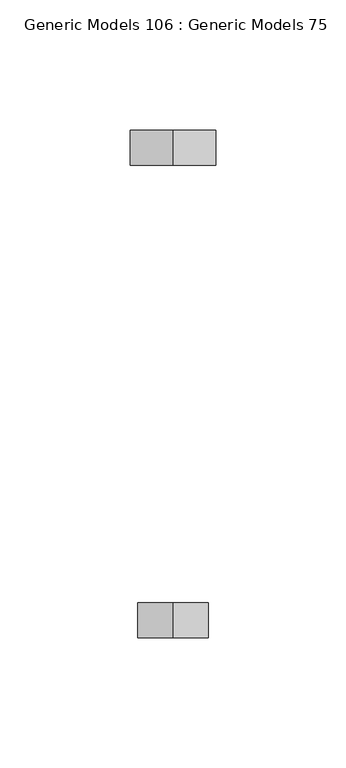
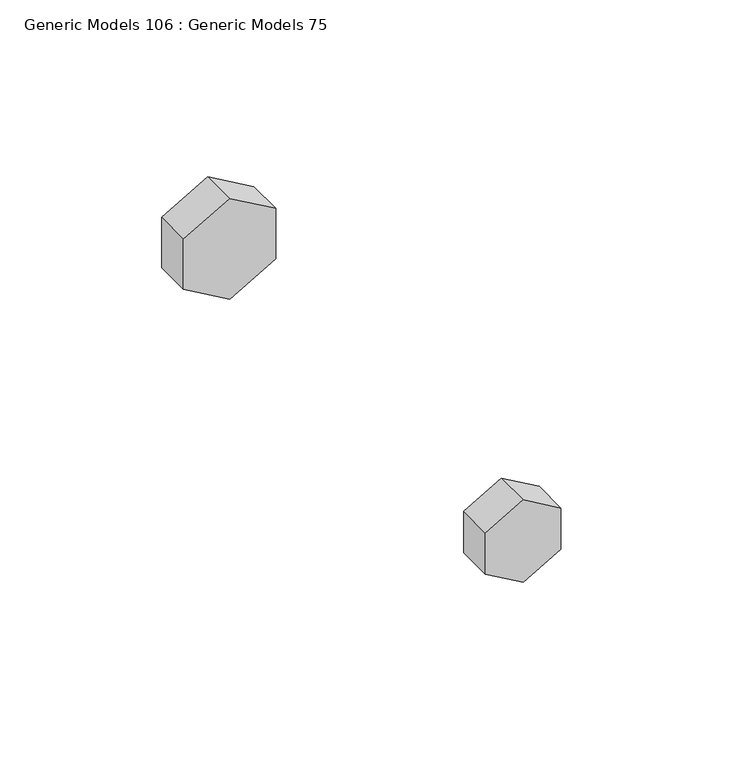
"""IFC4 building model written with IfcOpenShell, lengths in millimetres: proxy geometry, Generic Models 106 : Generic Models 75."""

from ifc_helpers import new_model, si_unit, frame, origin, place, context, project, spatial, polyline, outline, extrude, source, transform, mapped, element, save


def generic_models_106_generic_models_75_9fbede45(model_context):
    return source(origin(), model_context, "Body", "SweptSolid", [
        extrude(outline(polyline([(266588.875, 32004.6193618), (266607.925, 32004.6193618), (266617.45, 31988.1215778), (266607.925, 31971.6237939), (266588.875, 31971.6237939), (266579.35, 31988.1215778), (266588.875, 32004.6193618)])), frame((0.0, 36491.5582942, 0.0), z_axis=(0.0, 1.0, 0.0), x_axis=(0.0, 0.0, 1.0)), (0.0, 0.0, 1.0), 13.49375),
        extrude(outline(polyline([(266606.0078422, 31974.6312024), (266590.4304985, 31974.6312024), (266582.6418266, 31988.1215778), (266590.4304985, 32001.6119532), (266606.0078422, 32001.6119532), (266613.7965141, 31988.1215778), (266606.0078422, 31974.6312024)])), frame((0.0, 36309.7895442, 0.0), z_axis=(0.0, 1.0, 0.0), x_axis=(0.0, 0.0, 1.0)), (0.0, 0.0, 1.0), 13.49375),
    ])


if __name__ == "__main__":
    model = new_model("IFC4")
    model_context = context("Model", 3, world=origin())
    ifc_project = project(units=[si_unit("LENGTHUNIT", "METRE", prefix="MILLI")], contexts=[model_context])
    site = spatial("IfcSite", under=ifc_project)
    building = spatial("IfcBuilding", under=site)
    placement = place(None, origin())
    generic_models_106_generic_models_75_shape = generic_models_106_generic_models_75_9fbede45(model_context)
    element("IfcBuildingElementProxy", 1, Name="Generic Models 106 : Generic Models 75", ObjectType="Generic Models 106 : Generic Models 75", at=placement, inside=building, context=model_context, shape_type="MappedRepresentation", body=[
        mapped(generic_models_106_generic_models_75_shape, transform((0.0, 0.0, 0.0), x_axis=(1.0, 0.0, 0.0), y_axis=(0.0, 1.0, 0.0), z_axis=(0.0, 0.0, 1.0))),
    ])
    save(model, "model.ifc")

# Revit data of these elements
# Element 1 (IfcBuildingElementProxy, "Generic Models 106 : Generic Models 75")
#   Materials on its faces: "5/8\" GALV. THRU BOLTS"
# Materials
#   "5/8\" GALV. THRU BOLTS": class "Generic", colour RGB 255 0 255, transparency 0, Cost = 0
